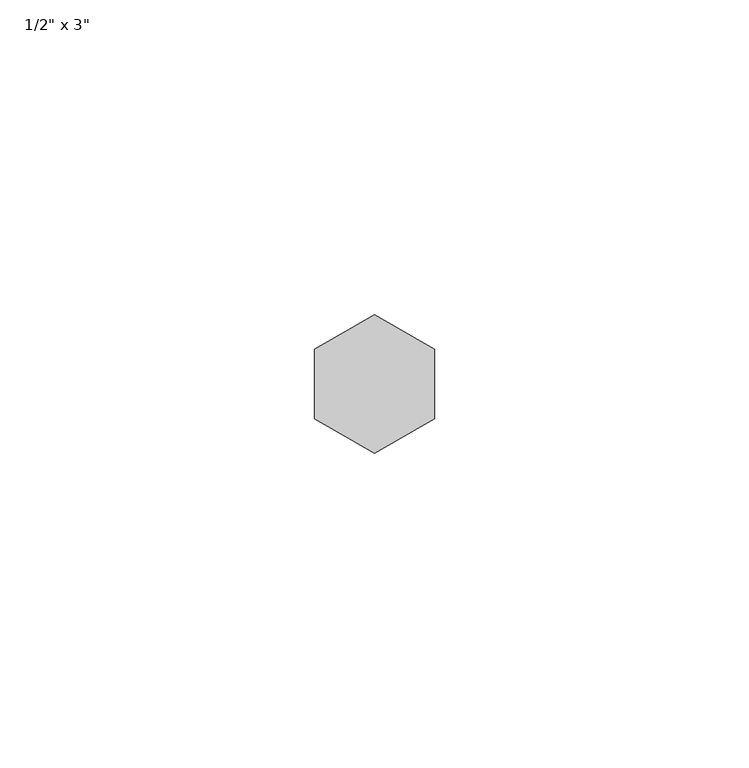
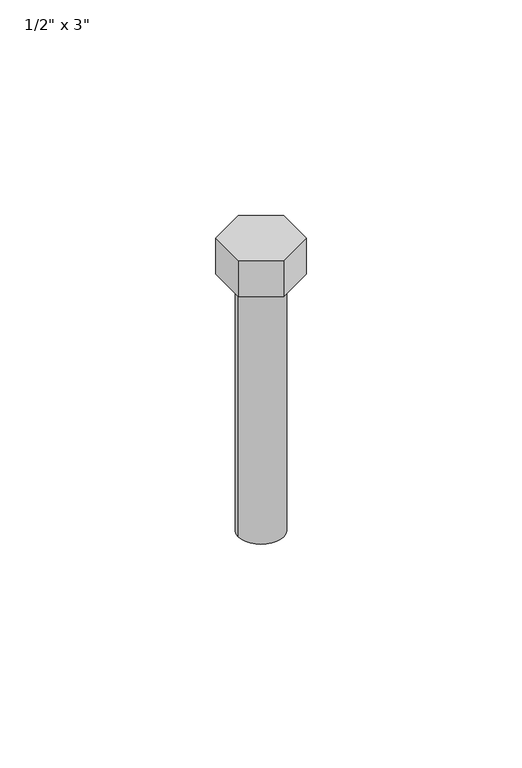
"""IFC4 building model written with IfcOpenShell, lengths in millimetres: proxy geometry."""

from ifc_helpers import new_model, si_unit, point, frame, origin, origin_with_axes, origin_2d, place, context, project, spatial, polyline, circle_curve, trimmed, segment, composite_curve, outline, extrude, source, transform, mapped, element, save


def proxy_435dac70(model_context):
    return source(origin(), model_context, "Body", "SweptSolid", [
        extrude(outline(polyline([(-9.525, 5.4992613), (0.0, 10.9985226), (9.525, 5.4992613), (9.525, -5.4992613), (0.0, -10.9985226), (-9.525, -5.4992613), (-9.525, 5.4992613)])), origin_with_axes(), (0.0, 0.0, 1.0), 10.715625),
        extrude(outline(composite_curve([segment(trimmed(circle_curve(origin_2d(), 6.35), [point((-6.35, 0.0))], [point((6.35, 0.0))], False, "CARTESIAN"), True, "CONTINUOUS"), segment(trimmed(circle_curve(origin_2d(), 6.35), [point((6.35, 0.0))], [point((-6.35, 0.0))], False, "CARTESIAN"), True, "CONTINUOUS")], self_intersect=False)), frame((0.0, 0.0, -76.2), z_axis=(0.0, 0.0, 1.0), x_axis=(1.0, 0.0, 0.0)), (0.0, 0.0, 1.0), 76.2),
    ])


if __name__ == "__main__":
    model = new_model("IFC4")
    model_context = context("Model", 3, world=origin())
    ifc_project = project(units=[si_unit("LENGTHUNIT", "METRE", prefix="MILLI")], contexts=[model_context])
    site = spatial("IfcSite", under=ifc_project)
    building = spatial("IfcBuilding", under=site)
    placement = place(None, origin())
    proxy_shape = proxy_435dac70(model_context)
    element("IfcBuildingElementProxy", 1, Name="050523 - W_P_C - Fastenings - Lag Bolt or Thru Bolt : 1/2\" x 3\"", ObjectType="050523 - W_P_C - Fastenings - Lag Bolt or Thru Bolt : 1/2\" x 3\"", at=placement, inside=building, context=model_context, shape_type="MappedRepresentation", body=[
        mapped(proxy_shape, transform((0.0, 0.0, 0.0), x_axis=(1.0, 0.0, 0.0), y_axis=(0.0, 1.0, 0.0), z_axis=(0.0, 0.0, 1.0))),
    ])
    save(model, "model.ifc")

# Revit data of these elements
# Type "050523 - W_P_C - Fastenings - Lag Bolt or Thru Bolt : 1/2\" x 3\""
#   Thickness_of_Substrate [instance default] = 0' - 1"
#   Side = 0' - 0 111/256"
#   Radius = 0' - 0 1/4"
#   Length = 0' - 3"
#   Head Size = 0' - 0 3/4"
#   Head Radius = 0' - 0 3/8"
#   Head Height = 0' - 0 27/64"
#   Diameter = 0' - 0 1/2"
#   Default Elevation = 4' - 0"
#   Nut_Visibility [instance default] = yes
#   Bolt Material (Size) = 1/2" DIA. A325 BOLT AT EACH PURLIN
# Element 1 (IfcBuildingElementProxy, "050523 - W_P_C - Fastenings - Lag Bolt or Thru Bolt : 1/2\" x 3\"")
#   Nut_Visibility = no
#   Materials on its faces: "1/2\" DIA. A325 BOLT AT EACH PURLIN"
# Materials
#   "1/2\" DIA. A325 BOLT AT EACH PURLIN": class "Generic", colour RGB 120 120 120, transparency 0, Cost = 0
